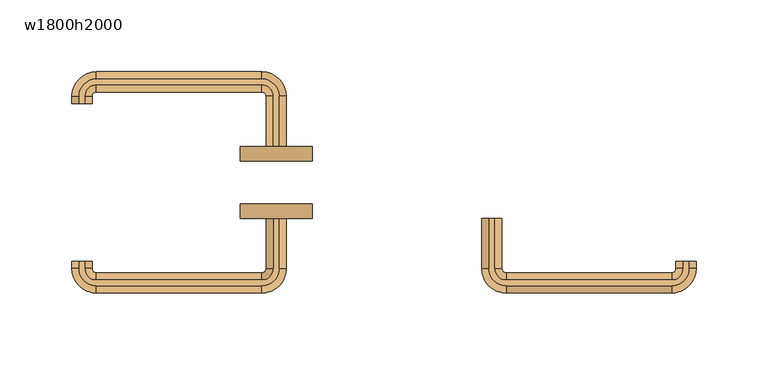
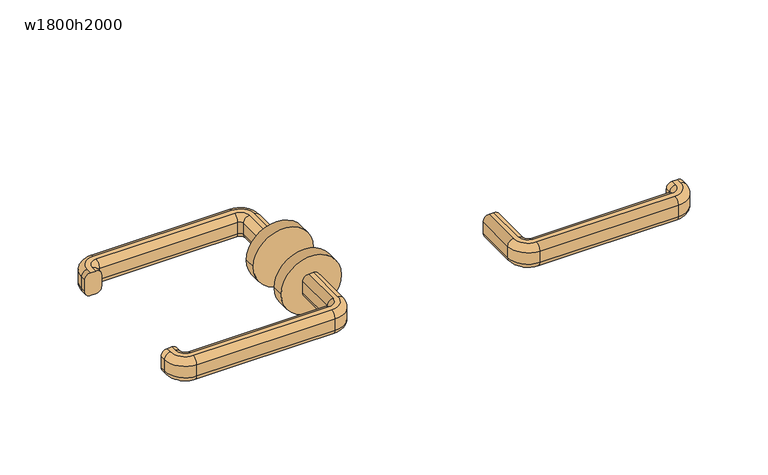
"""IFC4 building model written with IfcOpenShell, lengths in millimetres: door geometry, 二重 : w1800h2000."""

from ifc_helpers import new_model, si_unit, point, frame, frame_2d, origin, place, context, project, spatial, polyline, circle_curve, ellipse_curve, trimmed, segment, composite_curve, outline, extrude, source, transform, mapped, element, save
from ifc_brep_helpers import plane_surface, cylinder_surface, revolved_surface, advanced_brep


def w1800h2000_a1cd6a17(model_context):
    return source(origin(), model_context, "Body", "SolidModel", [
        advanced_brep(
        [(-73.0, -95.0, 960.0), (-68.0, -95.0, 955.0), (-68.0, -95.0, 945.0477623), (-73.0, -95.0, 940.0477623), (-77.0, -95.0, 940.0477623), (-82.0, -95.0, 945.0477623), (-82.0, -95.0, 955.0), (-77.0, -95.0, 960.0), (-73.0, -130.0, 960.0), (-68.0, -130.0, 955.0), (-68.0, -130.0, 945.0477623), (-73.0, -130.0, 940.0477623), (-85.0, -142.0, 940.0477623), (-200.0, -142.0, 940.0477623), (-212.0, -130.0, 940.0477623), (-212.0, -125.0, 940.0477623), (-208.0, -125.0, 940.0477623), (-208.0, -130.0, 940.0477623), (-200.0, -138.0, 940.0477623), (-85.0, -138.0, 940.0477623), (-77.0, -130.0, 940.0477623), (-82.0, -130.0, 945.0477623), (-82.0, -130.0, 955.0), (-77.0, -130.0, 960.0), (-85.0, -138.0, 960.0), (-200.0, -138.0, 960.0), (-208.0, -130.0, 960.0), (-208.0, -125.0, 960.0), (-212.0, -125.0, 960.0), (-212.0, -130.0, 960.0), (-200.0, -142.0, 960.0), (-85.0, -142.0, 960.0), (-85.0, -147.0, 955.0), (-85.0, -147.0, 945.0477623), (-85.0, -133.0, 945.0477623), (-85.0, -133.0, 955.0), (-200.0, -147.0, 955.0), (-200.0, -147.0, 945.0477623), (-200.0, -133.0, 945.0477623), (-200.0, -133.0, 955.0), (-217.0, -130.0, 955.0), (-217.0, -130.0, 945.0477623), (-203.0, -130.0, 945.0477623), (-203.0, -130.0, 955.0), (-203.0, -125.0, 955.0), (-203.0, -125.0, 945.0477623), (-217.0, -125.0, 945.0477623), (-217.0, -125.0, 955.0)],
        [
            (0, 1, circle_curve(frame((-73.0, -95.0, 955.0), z_axis=(0.0, 1.0, 0.0), x_axis=(1.0, 0.0, 0.0)), 5.0)),
            (1, 2),
            (2, 3, circle_curve(frame((-73.0, -95.0, 945.0477623), z_axis=(0.0, 1.0, 0.0), x_axis=(1.0, 0.0, 0.0)), 5.0)),
            (3, 4),
            (4, 5, circle_curve(frame((-77.0, -95.0, 945.0477623), z_axis=(0.0, 1.0, 0.0), x_axis=(1.0, 0.0, 0.0)), 5.0)),
            (5, 6),
            (6, 7, circle_curve(frame((-77.0, -95.0, 955.0), z_axis=(0.0, 1.0, 0.0), x_axis=(1.0, 0.0, 0.0)), 5.0)),
            (7, 0),
            (0, 8),
            (8, 9, circle_curve(frame((-73.0, -130.0, 955.0), z_axis=(0.0, 1.0, 0.0), x_axis=(1.0, 0.0, 0.0)), 5.0)),
            (9, 1),
            (9, 10),
            (10, 2),
            (10, 11, circle_curve(frame((-73.0, -130.0, 945.0477623), z_axis=(0.0, 1.0, 0.0), x_axis=(1.0, 0.0, 0.0)), 5.0)),
            (11, 3),
            (11, 12, circle_curve(frame((-85.0, -130.0, 940.0477623), z_axis=(0.0, 0.0, -1.0), x_axis=(1.0, 0.0, 0.0)), 12.0)),
            (12, 13),
            (13, 14, circle_curve(frame((-200.0, -130.0, 940.0477623), z_axis=(0.0, 0.0, -1.0), x_axis=(0.0, -1.0, 0.0)), 12.0)),
            (14, 15),
            (15, 16),
            (16, 17),
            (17, 18, circle_curve(frame((-200.0, -130.0, 940.0477623), z_axis=(0.0, 0.0, 1.0), x_axis=(0.0, -1.0, 0.0)), 8.0)),
            (18, 19),
            (19, 20, circle_curve(frame((-85.0, -130.0, 940.0477623), z_axis=(0.0, 0.0, 1.0), x_axis=(1.0, 0.0, 0.0)), 8.0)),
            (20, 4),
            (20, 21, circle_curve(frame((-77.0, -130.0, 945.0477623), z_axis=(0.0, 1.0, 0.0), x_axis=(1.0, 0.0, 0.0)), 5.0)),
            (21, 5),
            (21, 22),
            (22, 6),
            (22, 23, circle_curve(frame((-77.0, -130.0, 955.0), z_axis=(0.0, 1.0, 0.0), x_axis=(1.0, 0.0, 0.0)), 5.0)),
            (23, 7),
            (23, 24, circle_curve(frame((-85.0, -130.0, 960.0), z_axis=(0.0, 0.0, -1.0), x_axis=(1.0, 0.0, 0.0)), 8.0)),
            (24, 25),
            (25, 26, circle_curve(frame((-200.0, -130.0, 960.0), z_axis=(0.0, 0.0, -1.0), x_axis=(0.0, -1.0, 0.0)), 8.0)),
            (26, 27),
            (27, 28),
            (28, 29),
            (29, 30, circle_curve(frame((-200.0, -130.0, 960.0), z_axis=(0.0, 0.0, 1.0), x_axis=(0.0, -1.0, 0.0)), 12.0)),
            (30, 31),
            (31, 8, circle_curve(frame((-85.0, -130.0, 960.0), z_axis=(0.0, 0.0, 1.0), x_axis=(1.0, 0.0, 0.0)), 12.0)),
            (32, 9, circle_curve(frame((-85.0, -130.0, 955.0), z_axis=(0.0, 0.0, 1.0), x_axis=(1.0, 0.0, 0.0)), 17.0)),
            (31, 32, circle_curve(frame((-85.0, -142.0, 955.0), z_axis=(1.0, 0.0, 0.0), x_axis=(0.0, -1.0, 0.0)), 5.0)),
            (33, 10, circle_curve(frame((-85.0, -130.0, 945.0477623), z_axis=(0.0, 0.0, 1.0), x_axis=(1.0, 0.0, 0.0)), 17.0)),
            (32, 33),
            (33, 12, circle_curve(frame((-85.0, -142.0, 945.0477623), z_axis=(1.0, 0.0, 0.0), x_axis=(0.0, -1.0, 0.0)), 5.0)),
            (34, 21, circle_curve(frame((-85.0, -130.0, 945.0477623), z_axis=(0.0, 0.0, 1.0), x_axis=(1.0, 0.0, 0.0)), 3.0)),
            (19, 34, circle_curve(frame((-85.0, -138.0, 945.0477623), z_axis=(1.0, 0.0, 0.0), x_axis=(0.0, -1.0, 0.0)), 5.0)),
            (35, 22, circle_curve(frame((-85.0, -130.0, 955.0), z_axis=(0.0, 0.0, 1.0), x_axis=(1.0, 0.0, 0.0)), 3.0)),
            (34, 35),
            (35, 24, circle_curve(frame((-85.0, -138.0, 955.0), z_axis=(1.0, 0.0, 0.0), x_axis=(0.0, -1.0, 0.0)), 5.0)),
            (30, 36, circle_curve(frame((-200.0, -142.0, 955.0), z_axis=(1.0, 0.0, 0.0), x_axis=(0.0, -1.0, 0.0)), 5.0)),
            (36, 32),
            (36, 37),
            (37, 33),
            (37, 13, circle_curve(frame((-200.0, -142.0, 945.0477623), z_axis=(1.0, 0.0, 0.0), x_axis=(0.0, -1.0, 0.0)), 5.0)),
            (18, 38, circle_curve(frame((-200.0, -138.0, 945.0477623), z_axis=(1.0, 0.0, 0.0), x_axis=(0.0, -1.0, 0.0)), 5.0)),
            (38, 34),
            (38, 39),
            (39, 35),
            (39, 25, circle_curve(frame((-200.0, -138.0, 955.0), z_axis=(1.0, 0.0, 0.0), x_axis=(0.0, -1.0, 0.0)), 5.0)),
            (40, 36, circle_curve(frame((-200.0, -130.0, 955.0), z_axis=(0.0, 0.0, 1.0), x_axis=(0.0, -1.0, 0.0)), 17.0)),
            (29, 40, circle_curve(frame((-212.0, -130.0, 955.0), z_axis=(0.0, -1.0, 0.0), x_axis=(-1.0, 0.0, 0.0)), 5.0)),
            (41, 37, circle_curve(frame((-200.0, -130.0, 945.0477623), z_axis=(0.0, 0.0, 1.0), x_axis=(0.0, -1.0, 0.0)), 17.0)),
            (40, 41),
            (41, 14, circle_curve(frame((-212.0, -130.0, 945.0477623), z_axis=(0.0, -1.0, 0.0), x_axis=(-1.0, 0.0, 0.0)), 5.0)),
            (42, 38, circle_curve(frame((-200.0, -130.0, 945.0477623), z_axis=(0.0, 0.0, 1.0), x_axis=(0.0, -1.0, 0.0)), 3.0)),
            (17, 42, circle_curve(frame((-208.0, -130.0, 945.0477623), z_axis=(0.0, -1.0, 0.0), x_axis=(-1.0, 0.0, 0.0)), 5.0)),
            (43, 39, circle_curve(frame((-200.0, -130.0, 955.0), z_axis=(0.0, 0.0, 1.0), x_axis=(0.0, -1.0, 0.0)), 3.0)),
            (42, 43),
            (43, 26, circle_curve(frame((-208.0, -130.0, 955.0), z_axis=(0.0, -1.0, 0.0), x_axis=(-1.0, 0.0, 0.0)), 5.0)),
            (27, 44, circle_curve(frame((-208.0, -125.0, 955.0), z_axis=(0.0, 1.0, 0.0), x_axis=(-1.0, 0.0, 0.0)), 5.0)),
            (44, 45),
            (45, 16, circle_curve(frame((-208.0, -125.0, 945.0477623), z_axis=(0.0, 1.0, 0.0), x_axis=(-1.0, 0.0, 0.0)), 5.0)),
            (15, 46, circle_curve(frame((-212.0, -125.0, 945.0477623), z_axis=(0.0, 1.0, 0.0), x_axis=(-1.0, 0.0, 0.0)), 5.0)),
            (46, 47),
            (47, 28, circle_curve(frame((-212.0, -125.0, 955.0), z_axis=(0.0, 1.0, 0.0), x_axis=(-1.0, 0.0, 0.0)), 5.0)),
            (47, 40),
            (46, 41),
            (45, 42),
            (44, 43),
        ],
        [
            plane_surface(frame((-64.801961, -95.0, 950.0), z_axis=(0.0, 1.0, 0.0), x_axis=(0.0, 0.0, 1.0))),
            cylinder_surface(frame((-73.0, -95.0, 955.0), z_axis=(0.0, 1.0, 0.0), x_axis=(1.0, 0.0, 0.0)), 5.0),
            plane_surface(frame((-68.0, -95.0, 955.0), z_axis=(1.0, 0.0, 0.0), x_axis=(0.0, -1.0, 0.0))),
            cylinder_surface(frame((-73.0, -95.0, 945.0477623), z_axis=(0.0, 1.0, 0.0), x_axis=(1.0, 0.0, 0.0)), 5.0),
            plane_surface(frame((-73.0, -95.0, 940.0477623), z_axis=(0.0, 0.0, -1.0), x_axis=(0.0, -1.0, 0.0))),
            cylinder_surface(frame((-77.0, -95.0, 945.0477623), z_axis=(0.0, 1.0, 0.0), x_axis=(1.0, 0.0, 0.0)), 5.0),
            plane_surface(frame((-82.0, -95.0, 945.0477623), z_axis=(-1.0, 0.0, 0.0), x_axis=(0.0, -1.0, 0.0))),
            cylinder_surface(frame((-77.0, -95.0, 955.0), z_axis=(0.0, 1.0, 0.0), x_axis=(1.0, 0.0, 0.0)), 5.0),
            plane_surface(frame((-77.0, -95.0, 960.0), z_axis=(0.0, 0.0, 1.0), x_axis=(0.0, -1.0, 0.0))),
            revolved_surface(trimmed(ellipse_curve(frame((-73.0, -130.0, 955.0), z_axis=(0.0, 1.0, 0.0), x_axis=(1.0, 0.0, 0.0)), 5.0, 5.0), [point((-73.0, -130.0, 960.0))], [point((-68.0, -130.0, 955.0))], True, "CARTESIAN"), (-85.0, -130.0, 950.0), (0.0, 0.0, -1.0)),
            cylinder_surface(frame((-85.0, -130.0, 950.0), z_axis=(0.0, 0.0, -1.0), x_axis=(1.0, 0.0, 0.0)), 17.0),
            revolved_surface(trimmed(ellipse_curve(frame((-73.0, -130.0, 945.0477623), z_axis=(0.0, 1.0, 0.0), x_axis=(1.0, 0.0, 0.0)), 5.0, 5.0), [point((-68.0, -130.0, 945.0477623))], [point((-73.0, -130.0, 940.0477623))], True, "CARTESIAN"), (-85.0, -130.0, 950.0), (0.0, 0.0, -1.0)),
            revolved_surface(trimmed(ellipse_curve(frame((-77.0, -130.0, 945.0477623), z_axis=(0.0, 1.0, 0.0), x_axis=(1.0, 0.0, 0.0)), 5.0, 5.0), [point((-77.0, -130.0, 940.0477623))], [point((-82.0, -130.0, 945.0477623))], True, "CARTESIAN"), (-85.0, -130.0, 950.0), (0.0, 0.0, -1.0)),
            revolved_surface(polyline([(-82.0, -130.0, 945.0477623), (-82.0, -130.0, 955.0)]), (-85.0, -130.0, 950.0), (0.0, 0.0, -1.0)),
            revolved_surface(trimmed(ellipse_curve(frame((-77.0, -130.0, 955.0), z_axis=(0.0, 1.0, 0.0), x_axis=(1.0, 0.0, 0.0)), 5.0, 5.0), [point((-82.0, -130.0, 955.0))], [point((-77.0, -130.0, 960.0))], True, "CARTESIAN"), (-85.0, -130.0, 950.0), (0.0, 0.0, -1.0)),
            cylinder_surface(frame((-85.0, -142.0, 955.0), z_axis=(1.0, 0.0, 0.0), x_axis=(0.0, -1.0, 0.0)), 5.0),
            plane_surface(frame((-85.0, -147.0, 955.0), z_axis=(0.0, -1.0, 0.0), x_axis=(-1.0, 0.0, 0.0))),
            cylinder_surface(frame((-85.0, -142.0, 945.0477623), z_axis=(1.0, 0.0, 0.0), x_axis=(0.0, -1.0, 0.0)), 5.0),
            cylinder_surface(frame((-85.0, -138.0, 945.0477623), z_axis=(1.0, 0.0, 0.0), x_axis=(0.0, -1.0, 0.0)), 5.0),
            plane_surface(frame((-85.0, -133.0, 945.0477623), z_axis=(0.0, 1.0, 0.0), x_axis=(-1.0, 0.0, 0.0))),
            cylinder_surface(frame((-85.0, -138.0, 955.0), z_axis=(1.0, 0.0, 0.0), x_axis=(0.0, -1.0, 0.0)), 5.0),
            revolved_surface(trimmed(ellipse_curve(frame((-200.0, -142.0, 955.0), z_axis=(1.0, 0.0, 0.0), x_axis=(0.0, -1.0, 0.0)), 5.0, 5.0), [point((-200.0, -142.0, 960.0))], [point((-200.0, -147.0, 955.0))], True, "CARTESIAN"), (-200.0, -130.0, 950.0), (0.0, 0.0, -1.0)),
            cylinder_surface(frame((-200.0, -130.0, 950.0), z_axis=(0.0, 0.0, -1.0), x_axis=(0.0, -1.0, 0.0)), 17.0),
            revolved_surface(trimmed(ellipse_curve(frame((-200.0, -142.0, 945.0477623), z_axis=(1.0, 0.0, 0.0), x_axis=(0.0, -1.0, 0.0)), 5.0, 5.0), [point((-200.0, -147.0, 945.0477623))], [point((-200.0, -142.0, 940.0477623))], True, "CARTESIAN"), (-200.0, -130.0, 950.0), (0.0, 0.0, -1.0)),
            revolved_surface(trimmed(ellipse_curve(frame((-200.0, -138.0, 945.0477623), z_axis=(1.0, 0.0, 0.0), x_axis=(0.0, -1.0, 0.0)), 5.0, 5.0), [point((-200.0, -138.0, 940.0477623))], [point((-200.0, -133.0, 945.0477623))], True, "CARTESIAN"), (-200.0, -130.0, 950.0), (0.0, 0.0, -1.0)),
            revolved_surface(polyline([(-200.0, -133.0, 945.0477623), (-200.0, -133.0, 955.0)]), (-200.0, -130.0, 950.0), (0.0, 0.0, -1.0)),
            revolved_surface(trimmed(ellipse_curve(frame((-200.0, -138.0, 955.0), z_axis=(1.0, 0.0, 0.0), x_axis=(0.0, -1.0, 0.0)), 5.0, 5.0), [point((-200.0, -133.0, 955.0))], [point((-200.0, -138.0, 960.0))], True, "CARTESIAN"), (-200.0, -130.0, 950.0), (0.0, 0.0, -1.0)),
            plane_surface(frame((-199.801961, -125.0, 950.0), z_axis=(0.0, 1.0, 0.0), x_axis=(0.0, 0.0, -1.0))),
            cylinder_surface(frame((-212.0, -130.0, 955.0), z_axis=(0.0, -1.0, 0.0), x_axis=(-1.0, 0.0, 0.0)), 5.0),
            plane_surface(frame((-217.0, -130.0, 955.0), z_axis=(-1.0, 0.0, 0.0), x_axis=(0.0, 1.0, 0.0))),
            cylinder_surface(frame((-212.0, -130.0, 945.0477623), z_axis=(0.0, -1.0, 0.0), x_axis=(-1.0, 0.0, 0.0)), 5.0),
            cylinder_surface(frame((-208.0, -130.0, 945.0477623), z_axis=(0.0, -1.0, 0.0), x_axis=(-1.0, 0.0, 0.0)), 5.0),
            plane_surface(frame((-203.0, -130.0, 945.0477623), z_axis=(1.0, 0.0, 0.0), x_axis=(0.0, 1.0, 0.0))),
            cylinder_surface(frame((-208.0, -130.0, 955.0), z_axis=(0.0, -1.0, 0.0), x_axis=(-1.0, 0.0, 0.0)), 5.0),
        ],
        [
            (0, [[1, 2, 3, 4, 5, 6, 7, 8]]),
            (1, [[-1, 9, 10, 11]]),
            (2, [[-2, -11, 12, 13]]),
            (3, [[-3, -13, 14, 15]]),
            (4, [[-4, -15, 16, 17, 18, 19, 20, 21, 22, 23, 24, 25]]),
            (5, [[-5, -25, 26, 27]]),
            (6, [[-6, -27, 28, 29]]),
            (7, [[-7, -29, 30, 31]]),
            (8, [[-8, -31, 32, 33, 34, 35, 36, 37, 38, 39, 40, -9]]),
            (9, [[41, -10, -40, 42]]),
            (10, [[43, -12, -41, 44]]),
            (11, [[-16, -14, -43, 45]]),
            (12, [[46, -26, -24, 47]]),
            (13, [[48, -28, -46, 49]]),
            (14, [[-32, -30, -48, 50]]),
            (15, [[-42, -39, 51, 52]]),
            (16, [[-44, -52, 53, 54]]),
            (17, [[-45, -54, 55, -17]]),
            (18, [[-47, -23, 56, 57]]),
            (19, [[-49, -57, 58, 59]]),
            (20, [[-50, -59, 60, -33]]),
            (21, [[61, -51, -38, 62]]),
            (22, [[63, -53, -61, 64]]),
            (23, [[-18, -55, -63, 65]]),
            (24, [[66, -56, -22, 67]]),
            (25, [[68, -58, -66, 69]]),
            (26, [[-34, -60, -68, 70]]),
            (27, [[-36, 71, 72, 73, -20, 74, 75, 76]]),
            (28, [[-62, -37, -76, 77]]),
            (29, [[-64, -77, -75, 78]]),
            (30, [[-65, -78, -74, -19]]),
            (31, [[-67, -21, -73, 79]]),
            (32, [[-69, -79, -72, 80]]),
            (33, [[-70, -80, -71, -35]]),
        ],
    ),
        advanced_brep(
        [(-77.0, -45.0, 940.0), (-73.0, -45.0, 940.0), (-68.0, -45.0, 945.0), (-68.0, -45.0, 955.0), (-73.0, -45.0, 960.0), (-77.0, -45.0, 960.0), (-82.0, -45.0, 955.0), (-82.0, -45.0, 945.0), (-77.0, -10.0, 940.0), (-85.0, -2.0, 940.0), (-200.0, -2.0, 940.0), (-208.0, -10.0, 940.0), (-208.0, -15.0, 940.0), (-212.0, -15.0, 940.0), (-212.0, -10.0, 940.0), (-200.0, 2.0, 940.0), (-85.0, 2.0, 940.0), (-73.0, -10.0, 940.0), (-68.0, -10.0, 945.0), (-68.0, -10.0, 955.0), (-73.0, -10.0, 960.0), (-85.0, 2.0, 960.0), (-200.0, 2.0, 960.0), (-212.0, -10.0, 960.0), (-212.0, -15.0, 960.0), (-208.0, -15.0, 960.0), (-208.0, -10.0, 960.0), (-200.0, -2.0, 960.0), (-85.0, -2.0, 960.0), (-77.0, -10.0, 960.0), (-82.0, -10.0, 955.0), (-82.0, -10.0, 945.0), (-85.0, 7.0, 945.0), (-85.0, 7.0, 955.0), (-85.0, -7.0, 955.0), (-85.0, -7.0, 945.0), (-200.0, 7.0, 945.0), (-200.0, 7.0, 955.0), (-200.0, -7.0, 955.0), (-200.0, -7.0, 945.0), (-217.0, -10.0, 945.0), (-217.0, -10.0, 955.0), (-203.0, -10.0, 955.0), (-203.0, -10.0, 945.0), (-203.0, -15.0, 945.0), (-203.0, -15.0, 955.0), (-217.0, -15.0, 955.0), (-217.0, -15.0, 945.0)],
        [
            (0, 1),
            (1, 2, circle_curve(frame((-73.0, -45.0, 945.0), z_axis=(0.0, -1.0, 0.0), x_axis=(-1.0, 0.0, 0.0)), 5.0)),
            (2, 3),
            (3, 4, circle_curve(frame((-73.0, -45.0, 955.0), z_axis=(0.0, -1.0, 0.0), x_axis=(-1.0, 0.0, 0.0)), 5.0)),
            (4, 5),
            (5, 6, circle_curve(frame((-77.0, -45.0, 955.0), z_axis=(0.0, -1.0, 0.0), x_axis=(-1.0, 0.0, 0.0)), 5.0)),
            (6, 7),
            (7, 0, circle_curve(frame((-77.0, -45.0, 945.0), z_axis=(0.0, -1.0, 0.0), x_axis=(-1.0, 0.0, 0.0)), 5.0)),
            (0, 8),
            (8, 9, circle_curve(frame((-85.0, -10.0, 940.0), z_axis=(0.0, 0.0, 1.0), x_axis=(1.0, 0.0, 0.0)), 8.0)),
            (9, 10),
            (10, 11, circle_curve(frame((-200.0, -10.0, 940.0), z_axis=(0.0, 0.0, 1.0), x_axis=(0.0, 1.0, 0.0)), 8.0)),
            (11, 12),
            (12, 13),
            (13, 14),
            (14, 15, circle_curve(frame((-200.0, -10.0, 940.0), z_axis=(0.0, 0.0, -1.0), x_axis=(0.0, 1.0, 0.0)), 12.0)),
            (15, 16),
            (16, 17, circle_curve(frame((-85.0, -10.0, 940.0), z_axis=(0.0, 0.0, -1.0), x_axis=(1.0, 0.0, 0.0)), 12.0)),
            (17, 1),
            (17, 18, circle_curve(frame((-73.0, -10.0, 945.0), z_axis=(0.0, -1.0, 0.0), x_axis=(-1.0, 0.0, 0.0)), 5.0)),
            (18, 2),
            (18, 19),
            (19, 3),
            (19, 20, circle_curve(frame((-73.0, -10.0, 955.0), z_axis=(0.0, -1.0, 0.0), x_axis=(-1.0, 0.0, 0.0)), 5.0)),
            (20, 4),
            (20, 21, circle_curve(frame((-85.0, -10.0, 960.0), z_axis=(0.0, 0.0, 1.0), x_axis=(1.0, 0.0, 0.0)), 12.0)),
            (21, 22),
            (22, 23, circle_curve(frame((-200.0, -10.0, 960.0), z_axis=(0.0, 0.0, 1.0), x_axis=(0.0, 1.0, 0.0)), 12.0)),
            (23, 24),
            (24, 25),
            (25, 26),
            (26, 27, circle_curve(frame((-200.0, -10.0, 960.0), z_axis=(0.0, 0.0, -1.0), x_axis=(0.0, 1.0, 0.0)), 8.0)),
            (27, 28),
            (28, 29, circle_curve(frame((-85.0, -10.0, 960.0), z_axis=(0.0, 0.0, -1.0), x_axis=(1.0, 0.0, 0.0)), 8.0)),
            (29, 5),
            (29, 30, circle_curve(frame((-77.0, -10.0, 955.0), z_axis=(0.0, -1.0, 0.0), x_axis=(-1.0, 0.0, 0.0)), 5.0)),
            (30, 6),
            (30, 31),
            (31, 7),
            (31, 8, circle_curve(frame((-77.0, -10.0, 945.0), z_axis=(0.0, -1.0, 0.0), x_axis=(-1.0, 0.0, 0.0)), 5.0)),
            (32, 18, circle_curve(frame((-85.0, -10.0, 945.0), z_axis=(0.0, 0.0, -1.0), x_axis=(1.0, 0.0, 0.0)), 17.0)),
            (16, 32, circle_curve(frame((-85.0, 2.0, 945.0), z_axis=(1.0, 0.0, 0.0), x_axis=(0.0, -1.0, 0.0)), 5.0)),
            (33, 19, circle_curve(frame((-85.0, -10.0, 955.0), z_axis=(0.0, 0.0, -1.0), x_axis=(1.0, 0.0, 0.0)), 17.0)),
            (32, 33),
            (33, 21, circle_curve(frame((-85.0, 2.0, 955.0), z_axis=(1.0, 0.0, 0.0), x_axis=(0.0, -1.0, 0.0)), 5.0)),
            (34, 30, circle_curve(frame((-85.0, -10.0, 955.0), z_axis=(0.0, 0.0, -1.0), x_axis=(1.0, 0.0, 0.0)), 3.0)),
            (28, 34, circle_curve(frame((-85.0, -2.0, 955.0), z_axis=(1.0, 0.0, 0.0), x_axis=(0.0, -1.0, 0.0)), 5.0)),
            (35, 31, circle_curve(frame((-85.0, -10.0, 945.0), z_axis=(0.0, 0.0, -1.0), x_axis=(1.0, 0.0, 0.0)), 3.0)),
            (34, 35),
            (35, 9, circle_curve(frame((-85.0, -2.0, 945.0), z_axis=(1.0, 0.0, 0.0), x_axis=(0.0, -1.0, 0.0)), 5.0)),
            (15, 36, circle_curve(frame((-200.0, 2.0, 945.0), z_axis=(1.0, 0.0, 0.0), x_axis=(0.0, -1.0, 0.0)), 5.0)),
            (36, 32),
            (36, 37),
            (37, 33),
            (37, 22, circle_curve(frame((-200.0, 2.0, 955.0), z_axis=(1.0, 0.0, 0.0), x_axis=(0.0, -1.0, 0.0)), 5.0)),
            (27, 38, circle_curve(frame((-200.0, -2.0, 955.0), z_axis=(1.0, 0.0, 0.0), x_axis=(0.0, -1.0, 0.0)), 5.0)),
            (38, 34),
            (38, 39),
            (39, 35),
            (39, 10, circle_curve(frame((-200.0, -2.0, 945.0), z_axis=(1.0, 0.0, 0.0), x_axis=(0.0, -1.0, 0.0)), 5.0)),
            (40, 36, circle_curve(frame((-200.0, -10.0, 945.0), z_axis=(0.0, 0.0, -1.0), x_axis=(0.0, 1.0, 0.0)), 17.0)),
            (14, 40, circle_curve(frame((-212.0, -10.0, 945.0), z_axis=(0.0, 1.0, 0.0), x_axis=(1.0, 0.0, 0.0)), 5.0)),
            (41, 37, circle_curve(frame((-200.0, -10.0, 955.0), z_axis=(0.0, 0.0, -1.0), x_axis=(0.0, 1.0, 0.0)), 17.0)),
            (40, 41),
            (41, 23, circle_curve(frame((-212.0, -10.0, 955.0), z_axis=(0.0, 1.0, 0.0), x_axis=(1.0, 0.0, 0.0)), 5.0)),
            (42, 38, circle_curve(frame((-200.0, -10.0, 955.0), z_axis=(0.0, 0.0, -1.0), x_axis=(0.0, 1.0, 0.0)), 3.0)),
            (26, 42, circle_curve(frame((-208.0, -10.0, 955.0), z_axis=(0.0, 1.0, 0.0), x_axis=(1.0, 0.0, 0.0)), 5.0)),
            (43, 39, circle_curve(frame((-200.0, -10.0, 945.0), z_axis=(0.0, 0.0, -1.0), x_axis=(0.0, 1.0, 0.0)), 3.0)),
            (42, 43),
            (43, 11, circle_curve(frame((-208.0, -10.0, 945.0), z_axis=(0.0, 1.0, 0.0), x_axis=(1.0, 0.0, 0.0)), 5.0)),
            (12, 44, circle_curve(frame((-208.0, -15.0, 945.0), z_axis=(0.0, -1.0, 0.0), x_axis=(1.0, 0.0, 0.0)), 5.0)),
            (44, 45),
            (45, 25, circle_curve(frame((-208.0, -15.0, 955.0), z_axis=(0.0, -1.0, 0.0), x_axis=(1.0, 0.0, 0.0)), 5.0)),
            (24, 46, circle_curve(frame((-212.0, -15.0, 955.0), z_axis=(0.0, -1.0, 0.0), x_axis=(1.0, 0.0, 0.0)), 5.0)),
            (46, 47),
            (47, 13, circle_curve(frame((-212.0, -15.0, 945.0), z_axis=(0.0, -1.0, 0.0), x_axis=(1.0, 0.0, 0.0)), 5.0)),
            (47, 40),
            (46, 41),
            (45, 42),
            (44, 43),
        ],
        [
            plane_surface(frame((-64.801961, -45.0, 950.0), z_axis=(0.0, -1.0, 0.0), x_axis=(0.0, 0.0, -1.0))),
            plane_surface(frame((-77.0, -45.0, 940.0), z_axis=(0.0, 0.0, -1.0), x_axis=(0.0, 1.0, 0.0))),
            cylinder_surface(frame((-73.0, -45.0, 945.0), z_axis=(0.0, -1.0, 0.0), x_axis=(-1.0, 0.0, 0.0)), 5.0),
            plane_surface(frame((-68.0, -45.0, 945.0), z_axis=(1.0, 0.0, 0.0), x_axis=(0.0, 1.0, 0.0))),
            cylinder_surface(frame((-73.0, -45.0, 955.0), z_axis=(0.0, -1.0, 0.0), x_axis=(-1.0, 0.0, 0.0)), 5.0),
            plane_surface(frame((-73.0, -45.0, 960.0), z_axis=(0.0, 0.0, 1.0), x_axis=(0.0, 1.0, 0.0))),
            cylinder_surface(frame((-77.0, -45.0, 955.0), z_axis=(0.0, -1.0, 0.0), x_axis=(-1.0, 0.0, 0.0)), 5.0),
            plane_surface(frame((-82.0, -45.0, 955.0), z_axis=(-1.0, 0.0, 0.0), x_axis=(0.0, 1.0, 0.0))),
            cylinder_surface(frame((-77.0, -45.0, 945.0), z_axis=(0.0, -1.0, 0.0), x_axis=(-1.0, 0.0, 0.0)), 5.0),
            revolved_surface(trimmed(ellipse_curve(frame((-73.0, -10.0, 945.0), z_axis=(0.0, -1.0, 0.0), x_axis=(-1.0, 0.0, 0.0)), 5.0, 5.0), [point((-73.0, -10.0, 940.0))], [point((-68.0, -10.0, 945.0))], True, "CARTESIAN"), (-85.0, -10.0, 950.0), (0.0, 0.0, 1.0)),
            cylinder_surface(frame((-85.0, -10.0, 950.0), z_axis=(0.0, 0.0, 1.0), x_axis=(1.0, 0.0, 0.0)), 17.0),
            revolved_surface(trimmed(ellipse_curve(frame((-73.0, -10.0, 955.0), z_axis=(0.0, -1.0, 0.0), x_axis=(-1.0, 0.0, 0.0)), 5.0, 5.0), [point((-68.0, -10.0, 955.0))], [point((-73.0, -10.0, 960.0))], True, "CARTESIAN"), (-85.0, -10.0, 950.0), (0.0, 0.0, 1.0)),
            revolved_surface(trimmed(ellipse_curve(frame((-77.0, -10.0, 955.0), z_axis=(0.0, -1.0, 0.0), x_axis=(-1.0, 0.0, 0.0)), 5.0, 5.0), [point((-77.0, -10.0, 960.0))], [point((-82.0, -10.0, 955.0))], True, "CARTESIAN"), (-85.0, -10.0, 950.0), (0.0, 0.0, 1.0)),
            revolved_surface(polyline([(-82.0, -10.0, 955.0), (-82.0, -10.0, 945.0)]), (-85.0, -10.0, 950.0), (0.0, 0.0, 1.0)),
            revolved_surface(trimmed(ellipse_curve(frame((-77.0, -10.0, 945.0), z_axis=(0.0, -1.0, 0.0), x_axis=(-1.0, 0.0, 0.0)), 5.0, 5.0), [point((-82.0, -10.0, 945.0))], [point((-77.0, -10.0, 940.0))], True, "CARTESIAN"), (-85.0, -10.0, 950.0), (0.0, 0.0, 1.0)),
            cylinder_surface(frame((-85.0, 2.0, 945.0), z_axis=(1.0, 0.0, 0.0), x_axis=(0.0, -1.0, 0.0)), 5.0),
            plane_surface(frame((-85.0, 7.0, 945.0), z_axis=(0.0, 1.0, 0.0), x_axis=(-1.0, 0.0, 0.0))),
            cylinder_surface(frame((-85.0, 2.0, 955.0), z_axis=(1.0, 0.0, 0.0), x_axis=(0.0, -1.0, 0.0)), 5.0),
            cylinder_surface(frame((-85.0, -2.0, 955.0), z_axis=(1.0, 0.0, 0.0), x_axis=(0.0, -1.0, 0.0)), 5.0),
            plane_surface(frame((-85.0, -7.0, 955.0), z_axis=(0.0, -1.0, 0.0), x_axis=(-1.0, 0.0, 0.0))),
            cylinder_surface(frame((-85.0, -2.0, 945.0), z_axis=(1.0, 0.0, 0.0), x_axis=(0.0, -1.0, 0.0)), 5.0),
            revolved_surface(trimmed(ellipse_curve(frame((-200.0, 2.0, 945.0), z_axis=(1.0, 0.0, 0.0), x_axis=(0.0, -1.0, 0.0)), 5.0, 5.0), [point((-200.0, 2.0, 940.0))], [point((-200.0, 7.0, 945.0))], True, "CARTESIAN"), (-200.0, -10.0, 950.0), (0.0, 0.0, 1.0)),
            cylinder_surface(frame((-200.0, -10.0, 950.0), z_axis=(0.0, 0.0, 1.0), x_axis=(0.0, 1.0, 0.0)), 17.0),
            revolved_surface(trimmed(ellipse_curve(frame((-200.0, 2.0, 955.0), z_axis=(1.0, 0.0, 0.0), x_axis=(0.0, -1.0, 0.0)), 5.0, 5.0), [point((-200.0, 7.0, 955.0))], [point((-200.0, 2.0, 960.0))], True, "CARTESIAN"), (-200.0, -10.0, 950.0), (0.0, 0.0, 1.0)),
            revolved_surface(trimmed(ellipse_curve(frame((-200.0, -2.0, 955.0), z_axis=(1.0, 0.0, 0.0), x_axis=(0.0, -1.0, 0.0)), 5.0, 5.0), [point((-200.0, -2.0, 960.0))], [point((-200.0, -7.0, 955.0))], True, "CARTESIAN"), (-200.0, -10.0, 950.0), (0.0, 0.0, 1.0)),
            revolved_surface(polyline([(-200.0, -7.0, 955.0), (-200.0, -7.0, 945.0)]), (-200.0, -10.0, 950.0), (0.0, 0.0, 1.0)),
            revolved_surface(trimmed(ellipse_curve(frame((-200.0, -2.0, 945.0), z_axis=(1.0, 0.0, 0.0), x_axis=(0.0, -1.0, 0.0)), 5.0, 5.0), [point((-200.0, -7.0, 945.0))], [point((-200.0, -2.0, 940.0))], True, "CARTESIAN"), (-200.0, -10.0, 950.0), (0.0, 0.0, 1.0)),
            plane_surface(frame((-199.801961, -15.0, 950.0), z_axis=(0.0, -1.0, 0.0), x_axis=(0.0, 0.0, 1.0))),
            cylinder_surface(frame((-212.0, -10.0, 945.0), z_axis=(0.0, 1.0, 0.0), x_axis=(1.0, 0.0, 0.0)), 5.0),
            plane_surface(frame((-217.0, -10.0, 945.0), z_axis=(-1.0, 0.0, 0.0), x_axis=(0.0, -1.0, 0.0))),
            cylinder_surface(frame((-212.0, -10.0, 955.0), z_axis=(0.0, 1.0, 0.0), x_axis=(1.0, 0.0, 0.0)), 5.0),
            cylinder_surface(frame((-208.0, -10.0, 955.0), z_axis=(0.0, 1.0, 0.0), x_axis=(1.0, 0.0, 0.0)), 5.0),
            plane_surface(frame((-203.0, -10.0, 955.0), z_axis=(1.0, 0.0, 0.0), x_axis=(0.0, -1.0, 0.0))),
            cylinder_surface(frame((-208.0, -10.0, 945.0), z_axis=(0.0, 1.0, 0.0), x_axis=(1.0, 0.0, 0.0)), 5.0),
        ],
        [
            (0, [[1, 2, 3, 4, 5, 6, 7, 8]]),
            (1, [[-1, 9, 10, 11, 12, 13, 14, 15, 16, 17, 18, 19]]),
            (2, [[-2, -19, 20, 21]]),
            (3, [[-3, -21, 22, 23]]),
            (4, [[-4, -23, 24, 25]]),
            (5, [[-5, -25, 26, 27, 28, 29, 30, 31, 32, 33, 34, 35]]),
            (6, [[-6, -35, 36, 37]]),
            (7, [[-7, -37, 38, 39]]),
            (8, [[-8, -39, 40, -9]]),
            (9, [[41, -20, -18, 42]]),
            (10, [[43, -22, -41, 44]]),
            (11, [[-26, -24, -43, 45]]),
            (12, [[46, -36, -34, 47]]),
            (13, [[48, -38, -46, 49]]),
            (14, [[-10, -40, -48, 50]]),
            (15, [[-42, -17, 51, 52]]),
            (16, [[-44, -52, 53, 54]]),
            (17, [[-45, -54, 55, -27]]),
            (18, [[-47, -33, 56, 57]]),
            (19, [[-49, -57, 58, 59]]),
            (20, [[-50, -59, 60, -11]]),
            (21, [[61, -51, -16, 62]]),
            (22, [[63, -53, -61, 64]]),
            (23, [[-28, -55, -63, 65]]),
            (24, [[66, -56, -32, 67]]),
            (25, [[68, -58, -66, 69]]),
            (26, [[-12, -60, -68, 70]]),
            (27, [[71, 72, 73, -30, 74, 75, 76, -14]]),
            (28, [[-62, -15, -76, 77]]),
            (29, [[-64, -77, -75, 78]]),
            (30, [[-65, -78, -74, -29]]),
            (31, [[-67, -31, -73, 79]]),
            (32, [[-69, -79, -72, 80]]),
            (33, [[-70, -80, -71, -13]]),
        ],
    ),
        extrude(outline(composite_curve([segment(trimmed(circle_curve(frame_2d((950.0, -75.0)), 25.0), [point((950.0, -50.0))], [point((950.0, -100.0))], False, "CARTESIAN"), True, "CONTINUOUS"), segment(trimmed(circle_curve(frame_2d((950.0, -75.0)), 25.0), [point((950.0, -100.0))], [point((950.0, -50.0))], False, "CARTESIAN"), True, "CONTINUOUS")], self_intersect=False)), frame((0.0, -95.0, 0.0), z_axis=(0.0, 1.0, 0.0), x_axis=(0.0, 0.0, 1.0)), (0.0, 0.0, 1.0), 10.0),
        extrude(outline(composite_curve([segment(trimmed(circle_curve(frame_2d((950.0, -75.0)), 25.0), [point((950.0, -50.0))], [point((950.0, -100.0))], False, "CARTESIAN"), True, "CONTINUOUS"), segment(trimmed(circle_curve(frame_2d((950.0, -75.0)), 25.0), [point((950.0, -100.0))], [point((950.0, -50.0))], False, "CARTESIAN"), True, "CONTINUOUS")], self_intersect=False)), frame((0.0, -55.0, 0.0), z_axis=(0.0, 1.0, 0.0), x_axis=(0.0, 0.0, 1.0)), (0.0, 0.0, 1.0), 10.0),
        advanced_brep(
        [(73.0, -95.0, 960.0), (77.0, -95.0, 960.0), (82.0, -95.0, 955.0), (82.0, -95.0, 945.0477623), (77.0, -95.0, 940.0477623), (73.0, -95.0, 940.0477623), (68.0, -95.0, 945.0477623), (68.0, -95.0, 955.0), (68.0, -130.0, 955.0), (73.0, -130.0, 960.0), (68.0, -130.0, 945.0477623), (73.0, -130.0, 940.0477623), (77.0, -130.0, 940.0477623), (85.0, -138.0, 940.0477623), (200.0, -138.0, 940.0477623), (208.0, -130.0, 940.0477623), (208.0, -125.0, 940.0477623), (212.0, -125.0, 940.0477623), (212.0, -130.0, 940.0477623), (200.0, -142.0, 940.0477623), (85.0, -142.0, 940.0477623), (82.0, -130.0, 945.0477623), (82.0, -130.0, 955.0), (77.0, -130.0, 960.0), (85.0, -142.0, 960.0), (200.0, -142.0, 960.0), (212.0, -130.0, 960.0), (212.0, -125.0, 960.0), (208.0, -125.0, 960.0), (208.0, -130.0, 960.0), (200.0, -138.0, 960.0), (85.0, -138.0, 960.0), (85.0, -147.0, 955.0), (85.0, -147.0, 945.0477623), (85.0, -133.0, 945.0477623), (85.0, -133.0, 955.0), (200.0, -147.0, 955.0), (200.0, -147.0, 945.0477623), (200.0, -133.0, 945.0477623), (200.0, -133.0, 955.0), (217.0, -130.0, 955.0), (217.0, -130.0, 945.0477623), (203.0, -130.0, 945.0477623), (203.0, -130.0, 955.0), (217.0, -125.0, 955.0), (217.0, -125.0, 945.0477623), (203.0, -125.0, 945.0477623), (203.0, -125.0, 955.0)],
        [
            (0, 1),
            (1, 2, circle_curve(frame((77.0, -95.0, 955.0), z_axis=(0.0, 1.0, 0.0), x_axis=(-1.0, 0.0, 0.0)), 5.0)),
            (2, 3),
            (3, 4, circle_curve(frame((77.0, -95.0, 945.0477623), z_axis=(0.0, 1.0, 0.0), x_axis=(-1.0, 0.0, 0.0)), 5.0)),
            (4, 5),
            (5, 6, circle_curve(frame((73.0, -95.0, 945.0477623), z_axis=(0.0, 1.0, 0.0), x_axis=(-1.0, 0.0, 0.0)), 5.0)),
            (6, 7),
            (7, 0, circle_curve(frame((73.0, -95.0, 955.0), z_axis=(0.0, 1.0, 0.0), x_axis=(-1.0, 0.0, 0.0)), 5.0)),
            (7, 8),
            (8, 9, circle_curve(frame((73.0, -130.0, 955.0), z_axis=(0.0, 1.0, 0.0), x_axis=(-1.0, 0.0, 0.0)), 5.0)),
            (9, 0),
            (6, 10),
            (10, 8),
            (5, 11),
            (11, 10, circle_curve(frame((73.0, -130.0, 945.0477623), z_axis=(0.0, 1.0, 0.0), x_axis=(-1.0, 0.0, 0.0)), 5.0)),
            (4, 12),
            (12, 13, circle_curve(frame((85.0, -130.0, 940.0477623), z_axis=(0.0, 0.0, 1.0), x_axis=(-1.0, 0.0, 0.0)), 8.0)),
            (13, 14),
            (14, 15, circle_curve(frame((200.0, -130.0, 940.0477623), z_axis=(0.0, 0.0, 1.0), x_axis=(0.0, -1.0, 0.0)), 8.0)),
            (15, 16),
            (16, 17),
            (17, 18),
            (18, 19, circle_curve(frame((200.0, -130.0, 940.0477623), z_axis=(0.0, 0.0, -1.0), x_axis=(0.0, -1.0, 0.0)), 12.0)),
            (19, 20),
            (20, 11, circle_curve(frame((85.0, -130.0, 940.0477623), z_axis=(0.0, 0.0, -1.0), x_axis=(-1.0, 0.0, 0.0)), 12.0)),
            (3, 21),
            (21, 12, circle_curve(frame((77.0, -130.0, 945.0477623), z_axis=(0.0, 1.0, 0.0), x_axis=(-1.0, 0.0, 0.0)), 5.0)),
            (2, 22),
            (22, 21),
            (1, 23),
            (23, 22, circle_curve(frame((77.0, -130.0, 955.0), z_axis=(0.0, 1.0, 0.0), x_axis=(-1.0, 0.0, 0.0)), 5.0)),
            (9, 24, circle_curve(frame((85.0, -130.0, 960.0), z_axis=(0.0, 0.0, 1.0), x_axis=(-1.0, 0.0, 0.0)), 12.0)),
            (24, 25),
            (25, 26, circle_curve(frame((200.0, -130.0, 960.0), z_axis=(0.0, 0.0, 1.0), x_axis=(0.0, -1.0, 0.0)), 12.0)),
            (26, 27),
            (27, 28),
            (28, 29),
            (29, 30, circle_curve(frame((200.0, -130.0, 960.0), z_axis=(0.0, 0.0, -1.0), x_axis=(0.0, -1.0, 0.0)), 8.0)),
            (30, 31),
            (31, 23, circle_curve(frame((85.0, -130.0, 960.0), z_axis=(0.0, 0.0, -1.0), x_axis=(-1.0, 0.0, 0.0)), 8.0)),
            (32, 24, circle_curve(frame((85.0, -142.0, 955.0), z_axis=(-1.0, 0.0, 0.0), x_axis=(0.0, -1.0, 0.0)), 5.0)),
            (8, 32, circle_curve(frame((85.0, -130.0, 955.0), z_axis=(0.0, 0.0, 1.0), x_axis=(-1.0, 0.0, 0.0)), 17.0)),
            (33, 32),
            (10, 33, circle_curve(frame((85.0, -130.0, 945.0477623), z_axis=(0.0, 0.0, 1.0), x_axis=(-1.0, 0.0, 0.0)), 17.0)),
            (20, 33, circle_curve(frame((85.0, -142.0, 945.0477623), z_axis=(-1.0, 0.0, 0.0), x_axis=(0.0, -1.0, 0.0)), 5.0)),
            (34, 13, circle_curve(frame((85.0, -138.0, 945.0477623), z_axis=(-1.0, 0.0, 0.0), x_axis=(0.0, -1.0, 0.0)), 5.0)),
            (21, 34, circle_curve(frame((85.0, -130.0, 945.0477623), z_axis=(0.0, 0.0, 1.0), x_axis=(-1.0, 0.0, 0.0)), 3.0)),
            (35, 34),
            (22, 35, circle_curve(frame((85.0, -130.0, 955.0), z_axis=(0.0, 0.0, 1.0), x_axis=(-1.0, 0.0, 0.0)), 3.0)),
            (31, 35, circle_curve(frame((85.0, -138.0, 955.0), z_axis=(-1.0, 0.0, 0.0), x_axis=(0.0, -1.0, 0.0)), 5.0)),
            (32, 36),
            (36, 25, circle_curve(frame((200.0, -142.0, 955.0), z_axis=(-1.0, 0.0, 0.0), x_axis=(0.0, -1.0, 0.0)), 5.0)),
            (33, 37),
            (37, 36),
            (19, 37, circle_curve(frame((200.0, -142.0, 945.0477623), z_axis=(-1.0, 0.0, 0.0), x_axis=(0.0, -1.0, 0.0)), 5.0)),
            (34, 38),
            (38, 14, circle_curve(frame((200.0, -138.0, 945.0477623), z_axis=(-1.0, 0.0, 0.0), x_axis=(0.0, -1.0, 0.0)), 5.0)),
            (35, 39),
            (39, 38),
            (30, 39, circle_curve(frame((200.0, -138.0, 955.0), z_axis=(-1.0, 0.0, 0.0), x_axis=(0.0, -1.0, 0.0)), 5.0)),
            (40, 26, circle_curve(frame((212.0, -130.0, 955.0), z_axis=(0.0, -1.0, 0.0), x_axis=(1.0, 0.0, 0.0)), 5.0)),
            (36, 40, circle_curve(frame((200.0, -130.0, 955.0), z_axis=(0.0, 0.0, 1.0), x_axis=(0.0, -1.0, 0.0)), 17.0)),
            (41, 40),
            (37, 41, circle_curve(frame((200.0, -130.0, 945.0477623), z_axis=(0.0, 0.0, 1.0), x_axis=(0.0, -1.0, 0.0)), 17.0)),
            (18, 41, circle_curve(frame((212.0, -130.0, 945.0477623), z_axis=(0.0, -1.0, 0.0), x_axis=(1.0, 0.0, 0.0)), 5.0)),
            (42, 15, circle_curve(frame((208.0, -130.0, 945.0477623), z_axis=(0.0, -1.0, 0.0), x_axis=(1.0, 0.0, 0.0)), 5.0)),
            (38, 42, circle_curve(frame((200.0, -130.0, 945.0477623), z_axis=(0.0, 0.0, 1.0), x_axis=(0.0, -1.0, 0.0)), 3.0)),
            (43, 42),
            (39, 43, circle_curve(frame((200.0, -130.0, 955.0), z_axis=(0.0, 0.0, 1.0), x_axis=(0.0, -1.0, 0.0)), 3.0)),
            (29, 43, circle_curve(frame((208.0, -130.0, 955.0), z_axis=(0.0, -1.0, 0.0), x_axis=(1.0, 0.0, 0.0)), 5.0)),
            (27, 44, circle_curve(frame((212.0, -125.0, 955.0), z_axis=(0.0, 1.0, 0.0), x_axis=(1.0, 0.0, 0.0)), 5.0)),
            (44, 45),
            (45, 17, circle_curve(frame((212.0, -125.0, 945.0477623), z_axis=(0.0, 1.0, 0.0), x_axis=(1.0, 0.0, 0.0)), 5.0)),
            (16, 46, circle_curve(frame((208.0, -125.0, 945.0477623), z_axis=(0.0, 1.0, 0.0), x_axis=(1.0, 0.0, 0.0)), 5.0)),
            (46, 47),
            (47, 28, circle_curve(frame((208.0, -125.0, 955.0), z_axis=(0.0, 1.0, 0.0), x_axis=(1.0, 0.0, 0.0)), 5.0)),
            (40, 44),
            (41, 45),
            (42, 46),
            (43, 47),
        ],
        [
            plane_surface(frame((64.801961, -95.0, 950.0), z_axis=(0.0, 1.0, 0.0), x_axis=(0.0, 0.0, 1.0))),
            cylinder_surface(frame((73.0, -95.0, 955.0), z_axis=(0.0, 1.0, 0.0), x_axis=(-1.0, 0.0, 0.0)), 5.0),
            plane_surface(frame((68.0, -95.0, 955.0), z_axis=(-1.0, 0.0, 0.0), x_axis=(0.0, -1.0, 0.0))),
            cylinder_surface(frame((73.0, -95.0, 945.0477623), z_axis=(0.0, 1.0, 0.0), x_axis=(-1.0, 0.0, 0.0)), 5.0),
            plane_surface(frame((73.0, -95.0, 940.0477623), z_axis=(0.0, 0.0, -1.0), x_axis=(0.0, -1.0, 0.0))),
            cylinder_surface(frame((77.0, -95.0, 945.0477623), z_axis=(0.0, 1.0, 0.0), x_axis=(-1.0, 0.0, 0.0)), 5.0),
            plane_surface(frame((82.0, -95.0, 945.0477623), z_axis=(1.0, 0.0, 0.0), x_axis=(0.0, -1.0, 0.0))),
            cylinder_surface(frame((77.0, -95.0, 955.0), z_axis=(0.0, 1.0, 0.0), x_axis=(-1.0, 0.0, 0.0)), 5.0),
            plane_surface(frame((77.0, -95.0, 960.0), z_axis=(0.0, 0.0, 1.0), x_axis=(0.0, -1.0, 0.0))),
            revolved_surface(trimmed(ellipse_curve(frame((73.0, -130.0, 955.0), z_axis=(0.0, -1.0, 0.0), x_axis=(-1.0, 0.0, 0.0)), 5.0, 5.0), [point((73.0, -130.0, 960.0))], [point((68.0, -130.0, 955.0))], True, "CARTESIAN"), (85.0, -130.0, 950.0), (0.0, 0.0, -1.0)),
            cylinder_surface(frame((85.0, -130.0, 950.0), z_axis=(0.0, 0.0, -1.0), x_axis=(-1.0, 0.0, 0.0)), 17.0),
            revolved_surface(trimmed(ellipse_curve(frame((73.0, -130.0, 945.0477623), z_axis=(0.0, -1.0, 0.0), x_axis=(-1.0, 0.0, 0.0)), 5.0, 5.0), [point((68.0, -130.0, 945.0477623))], [point((73.0, -130.0, 940.0477623))], True, "CARTESIAN"), (85.0, -130.0, 950.0), (0.0, 0.0, -1.0)),
            revolved_surface(trimmed(ellipse_curve(frame((77.0, -130.0, 945.0477623), z_axis=(0.0, -1.0, 0.0), x_axis=(-1.0, 0.0, 0.0)), 5.0, 5.0), [point((77.0, -130.0, 940.0477623))], [point((82.0, -130.0, 945.0477623))], True, "CARTESIAN"), (85.0, -130.0, 950.0), (0.0, 0.0, -1.0)),
            revolved_surface(polyline([(82.0, -130.0, 945.0477623), (82.0, -130.0, 955.0)]), (85.0, -130.0, 950.0), (0.0, 0.0, -1.0)),
            revolved_surface(trimmed(ellipse_curve(frame((77.0, -130.0, 955.0), z_axis=(0.0, -1.0, 0.0), x_axis=(-1.0, 0.0, 0.0)), 5.0, 5.0), [point((82.0, -130.0, 955.0))], [point((77.0, -130.0, 960.0))], True, "CARTESIAN"), (85.0, -130.0, 950.0), (0.0, 0.0, -1.0)),
            cylinder_surface(frame((85.0, -142.0, 955.0), z_axis=(-1.0, 0.0, 0.0), x_axis=(0.0, -1.0, 0.0)), 5.0),
            plane_surface(frame((85.0, -147.0, 955.0), z_axis=(0.0, -1.0, 0.0), x_axis=(1.0, 0.0, 0.0))),
            cylinder_surface(frame((85.0, -142.0, 945.0477623), z_axis=(-1.0, 0.0, 0.0), x_axis=(0.0, -1.0, 0.0)), 5.0),
            cylinder_surface(frame((85.0, -138.0, 945.0477623), z_axis=(-1.0, 0.0, 0.0), x_axis=(0.0, -1.0, 0.0)), 5.0),
            plane_surface(frame((85.0, -133.0, 945.0477623), z_axis=(0.0, 1.0, 0.0), x_axis=(1.0, 0.0, 0.0))),
            cylinder_surface(frame((85.0, -138.0, 955.0), z_axis=(-1.0, 0.0, 0.0), x_axis=(0.0, -1.0, 0.0)), 5.0),
            revolved_surface(trimmed(ellipse_curve(frame((200.0, -142.0, 955.0), z_axis=(1.0, 0.0, 0.0), x_axis=(0.0, -1.0, 0.0)), 5.0, 5.0), [point((200.0, -142.0, 960.0))], [point((200.0, -147.0, 955.0))], True, "CARTESIAN"), (200.0, -130.0, 950.0), (0.0, 0.0, -1.0)),
            cylinder_surface(frame((200.0, -130.0, 950.0), z_axis=(0.0, 0.0, -1.0), x_axis=(0.0, -1.0, 0.0)), 17.0),
            revolved_surface(trimmed(ellipse_curve(frame((200.0, -142.0, 945.0477623), z_axis=(1.0, 0.0, 0.0), x_axis=(0.0, -1.0, 0.0)), 5.0, 5.0), [point((200.0, -147.0, 945.0477623))], [point((200.0, -142.0, 940.0477623))], True, "CARTESIAN"), (200.0, -130.0, 950.0), (0.0, 0.0, -1.0)),
            revolved_surface(trimmed(ellipse_curve(frame((200.0, -138.0, 945.0477623), z_axis=(1.0, 0.0, 0.0), x_axis=(0.0, -1.0, 0.0)), 5.0, 5.0), [point((200.0, -138.0, 940.0477623))], [point((200.0, -133.0, 945.0477623))], True, "CARTESIAN"), (200.0, -130.0, 950.0), (0.0, 0.0, -1.0)),
            revolved_surface(polyline([(200.0, -133.0, 945.0477623), (200.0, -133.0, 955.0)]), (200.0, -130.0, 950.0), (0.0, 0.0, -1.0)),
            revolved_surface(trimmed(ellipse_curve(frame((200.0, -138.0, 955.0), z_axis=(1.0, 0.0, 0.0), x_axis=(0.0, -1.0, 0.0)), 5.0, 5.0), [point((200.0, -133.0, 955.0))], [point((200.0, -138.0, 960.0))], True, "CARTESIAN"), (200.0, -130.0, 950.0), (0.0, 0.0, -1.0)),
            plane_surface(frame((199.801961, -125.0, 950.0), z_axis=(0.0, 1.0, 0.0), x_axis=(0.0, 0.0, -1.0))),
            cylinder_surface(frame((212.0, -130.0, 955.0), z_axis=(0.0, -1.0, 0.0), x_axis=(1.0, 0.0, 0.0)), 5.0),
            plane_surface(frame((217.0, -130.0, 955.0), z_axis=(1.0, 0.0, 0.0), x_axis=(0.0, 1.0, 0.0))),
            cylinder_surface(frame((212.0, -130.0, 945.0477623), z_axis=(0.0, -1.0, 0.0), x_axis=(1.0, 0.0, 0.0)), 5.0),
            cylinder_surface(frame((208.0, -130.0, 945.0477623), z_axis=(0.0, -1.0, 0.0), x_axis=(1.0, 0.0, 0.0)), 5.0),
            plane_surface(frame((203.0, -130.0, 945.0477623), z_axis=(-1.0, 0.0, 0.0), x_axis=(0.0, 1.0, 0.0))),
            cylinder_surface(frame((208.0, -130.0, 955.0), z_axis=(0.0, -1.0, 0.0), x_axis=(1.0, 0.0, 0.0)), 5.0),
        ],
        [
            (0, [[1, 2, 3, 4, 5, 6, 7, 8]]),
            (1, [[9, 10, 11, -8]]),
            (2, [[12, 13, -9, -7]]),
            (3, [[14, 15, -12, -6]]),
            (4, [[16, 17, 18, 19, 20, 21, 22, 23, 24, 25, -14, -5]]),
            (5, [[26, 27, -16, -4]]),
            (6, [[28, 29, -26, -3]]),
            (7, [[30, 31, -28, -2]]),
            (8, [[-11, 32, 33, 34, 35, 36, 37, 38, 39, 40, -30, -1]]),
            (9, [[41, -32, -10, 42]]),
            (10, [[43, -42, -13, 44]]),
            (11, [[45, -44, -15, -25]]),
            (12, [[46, -17, -27, 47]]),
            (13, [[48, -47, -29, 49]]),
            (14, [[50, -49, -31, -40]]),
            (15, [[51, 52, -33, -41]]),
            (16, [[53, 54, -51, -43]]),
            (17, [[-24, 55, -53, -45]]),
            (18, [[56, 57, -18, -46]]),
            (19, [[58, 59, -56, -48]]),
            (20, [[-39, 60, -58, -50]]),
            (21, [[61, -34, -52, 62]]),
            (22, [[63, -62, -54, 64]]),
            (23, [[65, -64, -55, -23]]),
            (24, [[66, -19, -57, 67]]),
            (25, [[68, -67, -59, 69]]),
            (26, [[70, -69, -60, -38]]),
            (27, [[71, 72, 73, -21, 74, 75, 76, -36]]),
            (28, [[77, -71, -35, -61]]),
            (29, [[78, -72, -77, -63]]),
            (30, [[-22, -73, -78, -65]]),
            (31, [[79, -74, -20, -66]]),
            (32, [[80, -75, -79, -68]]),
            (33, [[-37, -76, -80, -70]]),
        ],
    ),
    ])


if __name__ == "__main__":
    model = new_model("IFC4")
    model_context = context("Model", 3, world=origin())
    ifc_project = project(units=[si_unit("LENGTHUNIT", "METRE", prefix="MILLI")], contexts=[model_context])
    site = spatial("IfcSite", under=ifc_project)
    building = spatial("IfcBuilding", under=site)
    placement = place(None, origin())
    w1800h2000_shape = w1800h2000_a1cd6a17(model_context)
    element("IfcDoor", 1, ObjectType="二重 : w1800h2000", at=placement, inside=building, context=model_context, shape_type="MappedRepresentation", body=[
        mapped(w1800h2000_shape, transform((0.0, 0.0, 0.0), x_axis=(1.0, 0.0, 0.0), y_axis=(0.0, 1.0, 0.0), z_axis=(0.0, 0.0, 1.0))),
    ])
    save(model, "model.ifc")

# Revit data of these elements
# Type "二重 : w1800h2000"
#   Construction Type Id = "MDOOR"
#   Analytic Construction = "メタル"
#   Type Mark = "45"
#   Operation = "両開きドア単一スイング"
#   Keynote = "08110.R1"
#   Visual Light Transmittance = 0
#   Solar Heat Gain Coefficient = 0
#   Heat Transfer Coefficient (U) = 3.7021 W/(m²·K)
#   高さ(中心) = 1000 mm
#   Height = 2000 mm
#   Thickness = 30 mm
#   ドア枠見附 = 20 mm
#   Width = 1800 mm
#   取手取付け高さ = 950 mm
#   ドア枠ちり = 10 mm
#   Function = 0
#   ドア枠 [instance default] = none
#   ドア把手 [instance default] = メタル-ステンレス
#   ドア [instance default] = none
#   Wall Closure = (empty or 0)
# Element 1 (IfcDoor, "二重 : w1800h2000")
#   Materials on its faces: "メタル-ステンレス"
# Materials
#   "メタル-ステンレス": class "メタル", colour RGB 247 247 247, transparency 0, Cost = 0
